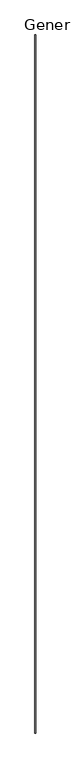
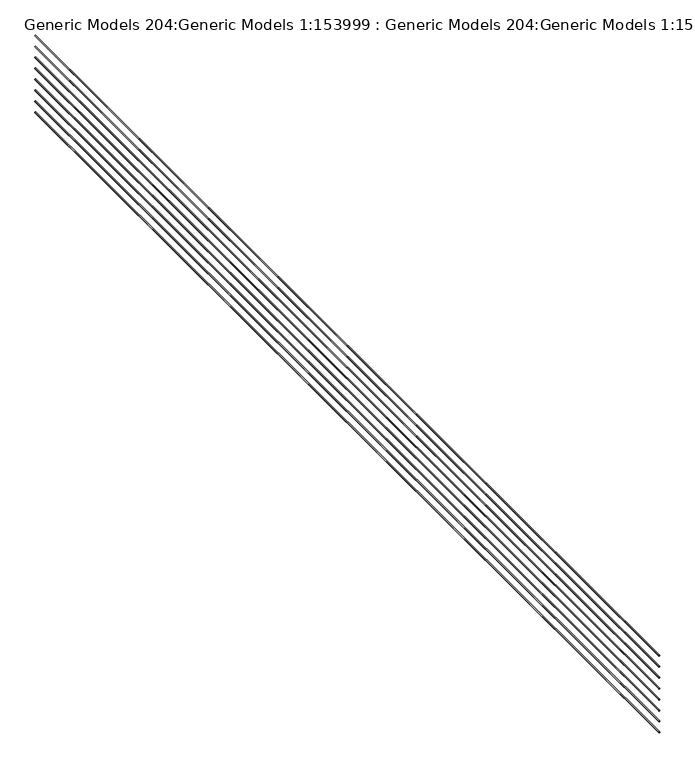
"""IFC4 building model written with IfcOpenShell, lengths in millimetres: proxy geometry, Generic Models 204:Generic Models 1:153999 : Generic Models 204:Generic Models 1:153999."""

from ifc_helpers import new_model, si_unit, point, frame, frame_2d, origin, place, context, project, spatial, circle_curve, trimmed, segment, composite_curve, outline, extrude, source, transform, mapped, element, save


def generic_models_204_generic_models_1_153999_generic_models_c4f67d17(model_context):
    return source(origin(), model_context, "Body", "SweptSolid", [
        extrude(outline(composite_curve([segment(trimmed(circle_curve(frame_2d((3743.325, -8296.396787)), 4.7625), [point((3743.325, -8301.159287))], [point((3743.325, -8291.634287))], False, "CARTESIAN"), True, "CONTINUOUS"), segment(trimmed(circle_curve(frame_2d((3743.325, -8296.396787)), 4.7625), [point((3743.325, -8291.634287))], [point((3743.325, -8301.159287))], False, "CARTESIAN"), True, "CONTINUOUS")], self_intersect=False)), frame((0.0, -464.4974793, 0.0), z_axis=(0.0, 1.0, 0.0), x_axis=(0.0, 0.0, 1.0)), (0.0, 0.0, 1.0), 9475.7774227),
        extrude(outline(composite_curve([segment(trimmed(circle_curve(frame_2d((3844.925, -8296.396787)), 4.7625), [point((3844.925, -8301.159287))], [point((3844.925, -8291.634287))], False, "CARTESIAN"), True, "CONTINUOUS"), segment(trimmed(circle_curve(frame_2d((3844.925, -8296.396787)), 4.7625), [point((3844.925, -8291.634287))], [point((3844.925, -8301.159287))], False, "CARTESIAN"), True, "CONTINUOUS")], self_intersect=False)), frame((0.0, -464.4974793, 0.0), z_axis=(0.0, 1.0, 0.0), x_axis=(0.0, 0.0, 1.0)), (0.0, 0.0, 1.0), 9475.7774227),
        extrude(outline(composite_curve([segment(trimmed(circle_curve(frame_2d((3946.525, -8296.396787)), 4.7625), [point((3946.525, -8301.159287))], [point((3946.525, -8291.634287))], False, "CARTESIAN"), True, "CONTINUOUS"), segment(trimmed(circle_curve(frame_2d((3946.525, -8296.396787)), 4.7625), [point((3946.525, -8291.634287))], [point((3946.525, -8301.159287))], False, "CARTESIAN"), True, "CONTINUOUS")], self_intersect=False)), frame((0.0, -464.4974793, 0.0), z_axis=(0.0, 1.0, 0.0), x_axis=(0.0, 0.0, 1.0)), (0.0, 0.0, 1.0), 9475.7774227),
        extrude(outline(composite_curve([segment(trimmed(circle_curve(frame_2d((4048.125, -8296.396787)), 4.7625), [point((4048.125, -8301.159287))], [point((4048.125, -8291.634287))], False, "CARTESIAN"), True, "CONTINUOUS"), segment(trimmed(circle_curve(frame_2d((4048.125, -8296.396787)), 4.7625), [point((4048.125, -8291.634287))], [point((4048.125, -8301.159287))], False, "CARTESIAN"), True, "CONTINUOUS")], self_intersect=False)), frame((0.0, -464.4974793, 0.0), z_axis=(0.0, 1.0, 0.0), x_axis=(0.0, 0.0, 1.0)), (0.0, 0.0, 1.0), 9475.7774227),
        extrude(outline(composite_curve([segment(trimmed(circle_curve(frame_2d((4149.725, -8296.396787)), 4.7625), [point((4149.725, -8301.159287))], [point((4149.725, -8291.634287))], False, "CARTESIAN"), True, "CONTINUOUS"), segment(trimmed(circle_curve(frame_2d((4149.725, -8296.396787)), 4.7625), [point((4149.725, -8291.634287))], [point((4149.725, -8301.159287))], False, "CARTESIAN"), True, "CONTINUOUS")], self_intersect=False)), frame((0.0, -464.4974793, 0.0), z_axis=(0.0, 1.0, 0.0), x_axis=(0.0, 0.0, 1.0)), (0.0, 0.0, 1.0), 9475.7774227),
        extrude(outline(composite_curve([segment(trimmed(circle_curve(frame_2d((4251.325, -8296.396787)), 4.7625), [point((4251.325, -8301.159287))], [point((4251.325, -8291.634287))], False, "CARTESIAN"), True, "CONTINUOUS"), segment(trimmed(circle_curve(frame_2d((4251.325, -8296.396787)), 4.7625), [point((4251.325, -8291.634287))], [point((4251.325, -8301.159287))], False, "CARTESIAN"), True, "CONTINUOUS")], self_intersect=False)), frame((0.0, -464.4974793, 0.0), z_axis=(0.0, 1.0, 0.0), x_axis=(0.0, 0.0, 1.0)), (0.0, 0.0, 1.0), 9475.7774227),
        extrude(outline(composite_curve([segment(trimmed(circle_curve(frame_2d((4352.925, -8296.396787)), 4.7625), [point((4352.925, -8301.159287))], [point((4352.925, -8291.634287))], False, "CARTESIAN"), True, "CONTINUOUS"), segment(trimmed(circle_curve(frame_2d((4352.925, -8296.396787)), 4.7625), [point((4352.925, -8291.634287))], [point((4352.925, -8301.159287))], False, "CARTESIAN"), True, "CONTINUOUS")], self_intersect=False)), frame((0.0, -464.4974793, 0.0), z_axis=(0.0, 1.0, 0.0), x_axis=(0.0, 0.0, 1.0)), (0.0, 0.0, 1.0), 9475.7774227),
        extrude(outline(composite_curve([segment(trimmed(circle_curve(frame_2d((4454.525, -8296.396787)), 4.7625), [point((4454.525, -8301.159287))], [point((4454.525, -8291.634287))], False, "CARTESIAN"), True, "CONTINUOUS"), segment(trimmed(circle_curve(frame_2d((4454.525, -8296.396787)), 4.7625), [point((4454.525, -8291.634287))], [point((4454.525, -8301.159287))], False, "CARTESIAN"), True, "CONTINUOUS")], self_intersect=False)), frame((0.0, -464.4974793, 0.0), z_axis=(0.0, 1.0, 0.0), x_axis=(0.0, 0.0, 1.0)), (0.0, 0.0, 1.0), 9475.7774227),
    ])


if __name__ == "__main__":
    model = new_model("IFC4")
    model_context = context("Model", 3, world=origin())
    ifc_project = project(units=[si_unit("LENGTHUNIT", "METRE", prefix="MILLI")], contexts=[model_context])
    site = spatial("IfcSite", under=ifc_project)
    building = spatial("IfcBuilding", under=site)
    placement = place(None, origin())
    generic_models_204_generic_models_1_153999_generic_models_shape = generic_models_204_generic_models_1_153999_generic_models_c4f67d17(model_context)
    element("IfcBuildingElementProxy", 1, Name="Generic Models 204:Generic Models 1:153999 : Generic Models 204:Generic Models 1:153999", ObjectType="Generic Models 204:Generic Models 1:153999 : Generic Models 204:Generic Models 1:153999", at=placement, inside=building, context=model_context, shape_type="MappedRepresentation", body=[
        mapped(generic_models_204_generic_models_1_153999_generic_models_shape, transform((0.0, 0.0, 0.0), x_axis=(1.0, 0.0, 0.0), y_axis=(0.0, 1.0, 0.0), z_axis=(0.0, 0.0, 1.0))),
    ])
    save(model, "model.ifc")

# Revit data of these elements
# Type "Generic Models 204:Generic Models 1:153999 : Generic Models 204:Generic Models 1:153999"
#   NameOverride = "Generic Models 204:Generic Models 1:153999"
#   ObjectTypeOverride = "Generic Models 204:Generic Models 1"
#   Reference = "Generic Models 1"
#   Category = "Generic Models"
#   Tag = "153999"
# Element 1 (IfcBuildingElementProxy, "Generic Models 204:Generic Models 1:153999 : Generic Models 204:Generic Models 1:153999")
#   Materials on its faces: "_1/2\" DIA. SOLID STOCK STEEL HORIZONTAL RAILINGS"
# Materials
#   "_1/2\" DIA. SOLID STOCK STEEL HORIZONTAL RAILINGS": class "Metal", colour RGB 199 199 199, transparency 0, Description = "Structural steel 50ksi", Cost = 0
